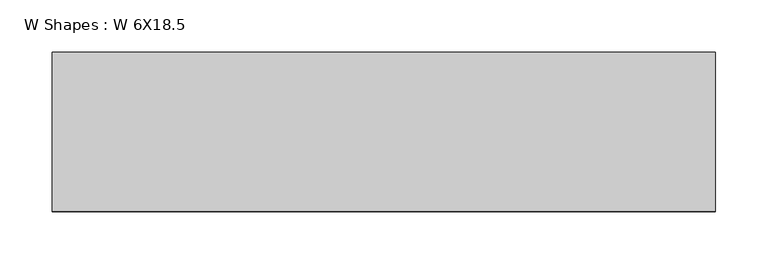
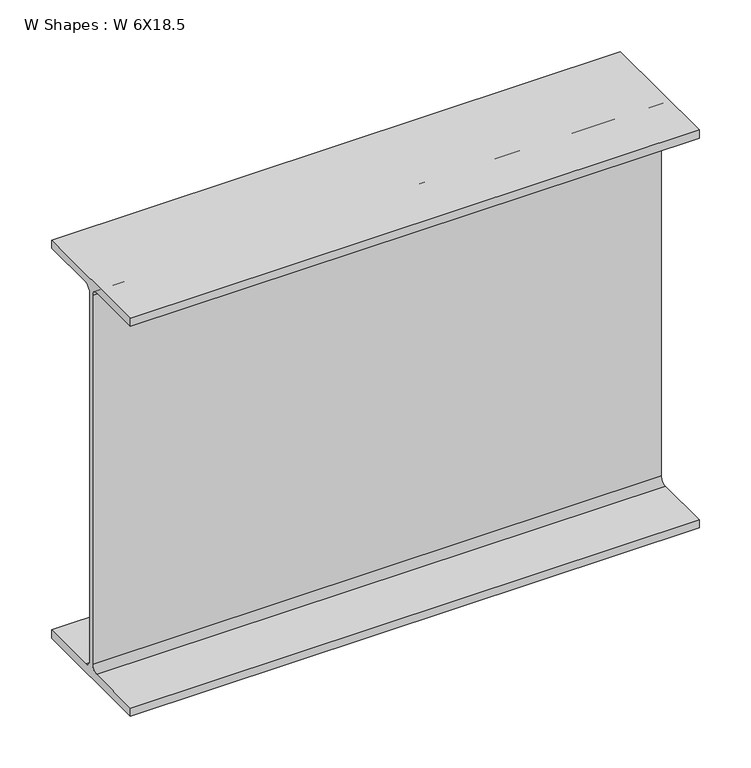
"""IFC4 building model written with IfcOpenShell, lengths in millimetres: beam geometry, W Shapes : W 6X18.5."""

from ifc_helpers import new_model, si_unit, point, frame, frame_2d, origin, place, context, project, spatial, polyline, circle_curve, trimmed, segment, composite_curve, outline, extrude, source, transform, mapped, element, save


def w_shapes_w_6x18_5_26640f6b(model_context):
    return source(origin(), model_context, "Body", "SweptSolid", [
        extrude(outline(composite_curve([segment(polyline([(76.1964281, -225.298), (76.1964281, -234.95), (-76.2035719, -234.95), (-76.2035719, -225.298), (-10.5445719, -225.298)]), True, "CONTINUOUS"), segment(trimmed(circle_curve(frame_2d((-10.5445719, -217.678)), 7.62), [point((-10.5445719, -225.298))], [point((-2.9245719, -217.678))], True, "CARTESIAN"), True, "CONTINUOUS"), segment(polyline([(-2.9245719, -217.678), (-2.9245719, 217.678)]), True, "CONTINUOUS"), segment(trimmed(circle_curve(frame_2d((-10.5445719, 217.678)), 7.62), [point((-2.9245719, 217.678))], [point((-10.5445719, 225.298))], True, "CARTESIAN"), True, "CONTINUOUS"), segment(polyline([(-10.5445719, 225.298), (-76.2035719, 225.298), (-76.2035719, 234.95), (76.1964281, 234.95), (76.1964281, 225.298), (10.5374281, 225.298)]), True, "CONTINUOUS"), segment(trimmed(circle_curve(frame_2d((10.5374281, 217.678)), 7.62), [point((10.5374281, 225.298))], [point((2.9174281, 217.678))], True, "CARTESIAN"), True, "CONTINUOUS"), segment(polyline([(2.9174281, 217.678), (2.9174281, -217.678)]), True, "CONTINUOUS"), segment(trimmed(circle_curve(frame_2d((10.5374281, -217.678)), 7.62), [point((2.9174281, -217.678))], [point((10.5374281, -225.298))], True, "CARTESIAN"), True, "CONTINUOUS"), segment(polyline([(10.5374281, -225.298), (76.1964281, -225.298)]), True, "CONTINUOUS")], self_intersect=False)), frame((-317.5, 0.0, 0.0), z_axis=(1.0, 0.0, 0.0), x_axis=(0.0, 1.0, 0.0)), (0.0, 0.0, 1.0), 635.0),
    ])


if __name__ == "__main__":
    model = new_model("IFC4")
    model_context = context("Model", 3, world=origin())
    ifc_project = project(units=[si_unit("LENGTHUNIT", "METRE", prefix="MILLI")], contexts=[model_context])
    site = spatial("IfcSite", under=ifc_project)
    building = spatial("IfcBuilding", under=site)
    placement = place(None, origin())
    w_shapes_w_6x18_5_shape = w_shapes_w_6x18_5_26640f6b(model_context)
    element("IfcBeam", 1, ObjectType="W Shapes : W 6X18.5", at=placement, inside=building, context=model_context, shape_type="MappedRepresentation", body=[
        mapped(w_shapes_w_6x18_5_shape, transform((0.0, 0.0, 0.0), x_axis=(1.0, 0.0, 0.0), y_axis=(0.0, 1.0, 0.0), z_axis=(0.0, 0.0, 1.0))),
    ])
    save(model, "model.ifc")

# Revit data of these elements
# Type "W Shapes : W 6X18.5"
#   Section Name Key = "W12x26"
#   Assembly Code = "B10"
#   Width = 152.4 mm
#   Web Thickness = 5.842 mm
#   Web Fillet = 7.62 mm
#   Warping Constant = 163001.3 cm⁶
#   Torsional Moment of Inertia = 12.4869 cm⁴
#   Section Area = 7.65 in²
#   Plastic Modulus weak axis = 0.00472801 (stored number, unit not read)
#   Plastic Modulus strong axis = 0.0215278 (stored number, unit not read)
#   Perimeter = 15.0571 m²/m
#   Nominal Weight = 379.441 N/m
#   Moment of Inertia weak axis = 720.08 cm⁴
#   Moment of Inertia strong axis = 8491.12 cm⁴
#   Height = 469.9 mm
#   Flange Thickness = 9.652 mm
#   Elastic Modulus weak axis = 0.00309028 (stored number, unit not read)
#   Elastic Modulus strong axis = 0.0193287 (stored number, unit not read)
#   Centroid Vertical = 234.95 mm
#   Centroid Horizontal = 76.2 mm
#   Length [instance default] = 5' - 0"
#   Structural Material [instance default] = Steel ASTM A992
#   Principal Axes Angle = 0
# Element 1 (IfcBeam, "W Shapes : W 6X18.5")
#   Materials on its faces: "Steel ASTM A992"
# Materials
#   "Steel ASTM A992": class "Metal", colour RGB 189 187 185, transparency 0, Description = "Structural steel 50ksi", Cost = 0
